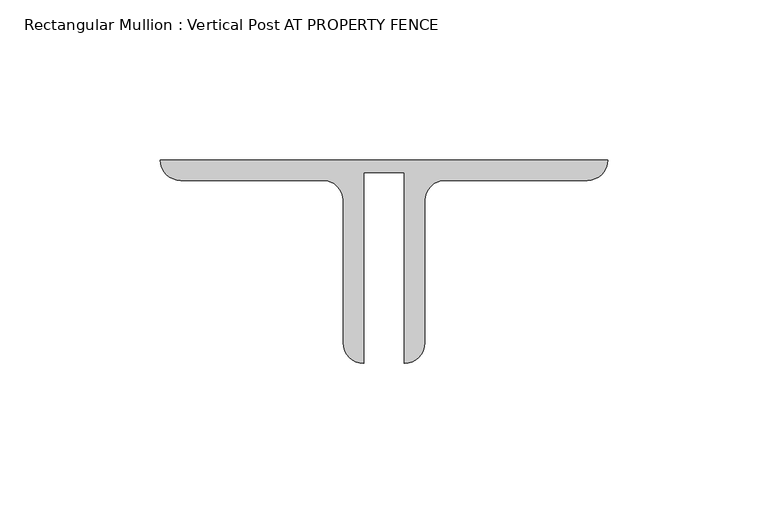
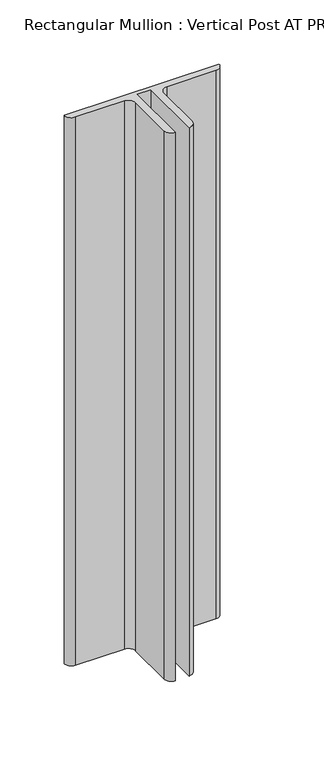
"""IFC4 building model written with IfcOpenShell, lengths in millimetres: member geometry, Rectangular Mullion : Vertical Post AT PROPERTY FENCE."""

from ifc_helpers import new_model, si_unit, point, frame, frame_2d, origin, place, context, project, spatial, polyline, circle_curve, trimmed, segment, composite_curve, outline, extrude, source, transform, mapped, element, save


def rectangular_mullion_vertical_post_at_property_fence_43cfa28e(model_context):
    return source(origin(), model_context, "Body", "SweptSolid", [
        extrude(outline(composite_curve([segment(polyline([(-6.35, -22.9145205), (-6.35, -82.55)]), True, "CONTINUOUS"), segment(trimmed(circle_curve(frame_2d((-6.35, -76.2)), 6.35), [point((-6.35, -82.55))], [point((-12.7, -76.2))], False, "CARTESIAN"), True, "CONTINUOUS"), segment(polyline([(-12.7, -76.2), (-12.7, -31.75)]), True, "CONTINUOUS"), segment(trimmed(circle_curve(frame_2d((-19.05, -31.75)), 6.35), [point((-12.7, -31.75))], [point((-19.05, -25.4))], True, "CARTESIAN"), True, "CONTINUOUS"), segment(polyline([(-19.05, -25.4), (-63.5, -25.4)]), True, "CONTINUOUS"), segment(trimmed(circle_curve(frame_2d((-63.5, -19.05)), 6.35), [point((-63.5, -25.4))], [point((-69.85, -19.05))], False, "CARTESIAN"), True, "CONTINUOUS"), segment(polyline([(-69.85, -19.05), (69.85, -19.05)]), True, "CONTINUOUS"), segment(trimmed(circle_curve(frame_2d((63.5, -19.05)), 6.35), [point((69.85, -19.05))], [point((63.5, -25.4))], False, "CARTESIAN"), True, "CONTINUOUS"), segment(polyline([(63.5, -25.4), (19.05, -25.4)]), True, "CONTINUOUS"), segment(trimmed(circle_curve(frame_2d((19.05, -31.75)), 6.35), [point((19.05, -25.4))], [point((12.7, -31.75))], True, "CARTESIAN"), True, "CONTINUOUS"), segment(polyline([(12.7, -31.75), (12.7, -76.2)]), True, "CONTINUOUS"), segment(trimmed(circle_curve(frame_2d((6.35, -76.2)), 6.35), [point((12.7, -76.2))], [point((6.35, -82.55))], False, "CARTESIAN"), True, "CONTINUOUS"), segment(polyline([(6.35, -82.55), (6.35, -22.9145205), (-6.35, -22.9145205)]), True, "CONTINUOUS")], self_intersect=False)), frame((0.0, 0.0, -522.9663052), z_axis=(0.0, 0.0, 1.0), x_axis=(1.0, 0.0, 0.0)), (0.0, 0.0, 1.0), 522.9663052),
    ])


if __name__ == "__main__":
    model = new_model("IFC4")
    model_context = context("Model", 3, world=origin())
    ifc_project = project(units=[si_unit("LENGTHUNIT", "METRE", prefix="MILLI")], contexts=[model_context])
    site = spatial("IfcSite", under=ifc_project)
    building = spatial("IfcBuilding", under=site)
    placement = place(None, origin())
    rectangular_mullion_vertical_post_at_property_fence_shape = rectangular_mullion_vertical_post_at_property_fence_43cfa28e(model_context)
    element("IfcMember", 1, ObjectType="Rectangular Mullion : Vertical Post AT PROPERTY FENCE", at=placement, inside=building, context=model_context, shape_type="MappedRepresentation", body=[
        mapped(rectangular_mullion_vertical_post_at_property_fence_shape, transform((0.0, 0.0, 0.0), x_axis=(1.0, 0.0, 0.0), y_axis=(0.0, 1.0, 0.0), z_axis=(0.0, 0.0, 1.0))),
    ])
    save(model, "model.ifc")

# Revit data of these elements
# Type "Rectangular Mullion : Vertical Post AT PROPERTY FENCE"
#   built-in parameter 1007351 = -0.0625 (stored number, unit not read)
#   built-in parameter 1007322 = 0.0126789 (stored number, unit not read)
#   built-in parameter 1007321 = 0.229167 (stored number, unit not read)
#   built-in parameter 1007320 = 0.229167 (stored number, unit not read)
# Element 1 (IfcMember, "Rectangular Mullion : Vertical Post AT PROPERTY FENCE")
#   Materials on its faces: "MAIN FENCE POST: (2) BACK/BACK GALVANIZED ANGLES (2) L2 1/2 X 2 1/2 X 1/4\") ANCHORED TO 8\"W X 42\" DEEP CONCRETE FOOTING(1)"
# Materials
#   "MAIN FENCE POST: (2) BACK/BACK GALVANIZED ANGLES (2) L2 1/2 X 2 1/2 X 1/4\") ANCHORED TO 8\"W X 42\" DEEP CONCRETE FOOTING(1)": class "Unassigned", colour RGB 211 211 211, transparency 0, Cost = 0
